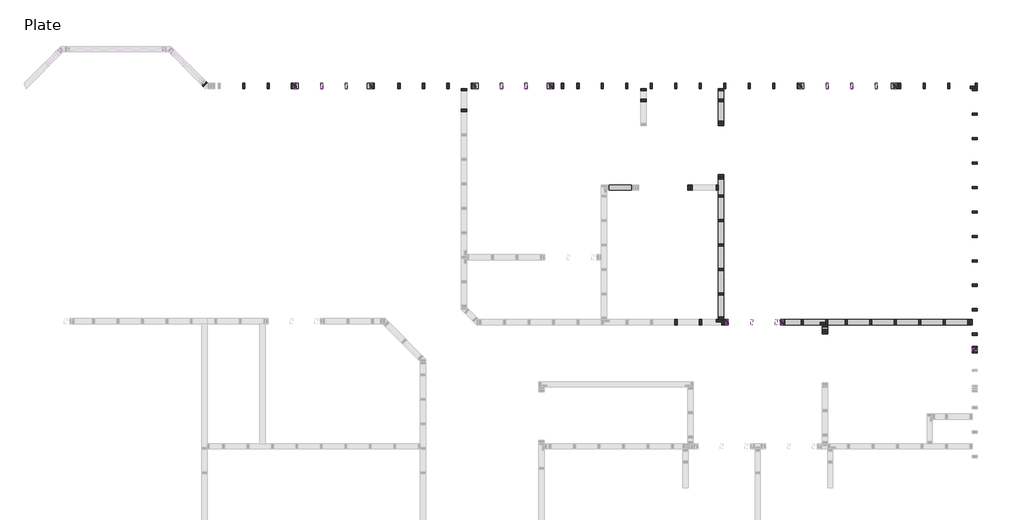
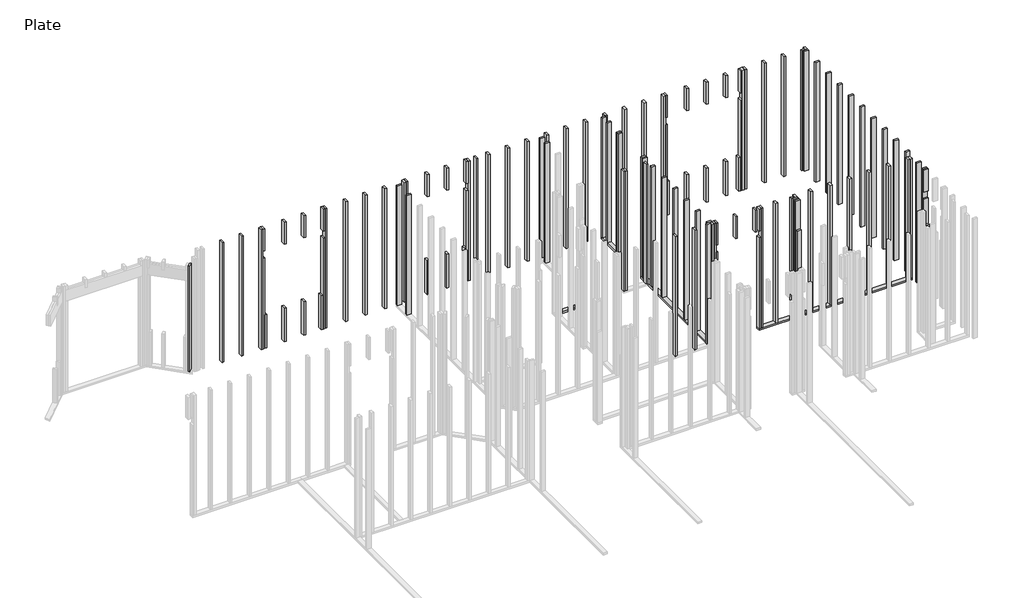
# One storey, part 5 of 5: 118 columns, 5 beams.
"""IFC4 building model written with IfcOpenShell, lengths in millimetres."""

import ifcopenshell
import ifcopenshell.guid

model = None  # the IFC model being written
_history = None  # IfcOwnerHistory: only IFC2X3 demands one
_inside = {}  # id of a spatial element -> (the spatial element, [elements in it])
_under = {}  # id of a project, library or spatial element -> (it, [spatial elements below it])
_declared = {}  # id of a project -> (the project, [libraries it declares])
_typed = {}  # id of a type object -> (the type object, [elements of that type])
_made_of = {}  # id of a material, layer set ... -> (it, [elements and type objects made of it])


def new_model(schema):
    """Start an empty IFC model of exactly this schema.

    Asked for "IFC4X3", IfcOpenShell would pick the latest addendum, in which some entities
    have other attributes; the version numbers below select the first issue.
    IFC2X3 requires an IfcOwnerHistory on every rooted entity: one is made here for all.
    """
    global model, _history
    if schema == "IFC4X3":
        model = ifcopenshell.file(schema_version=(4, 3, 0, 0))
    else:
        model = ifcopenshell.file(schema=schema)
    _inside.clear()
    _under.clear()
    _declared.clear()
    _typed.clear()
    _made_of.clear()
    _history = None
    if model.schema == "IFC2X3":
        org = make("IfcOrganization", Name="unknown")
        user = make(
            "IfcPersonAndOrganization",
            ThePerson=make("IfcPerson", FamilyName="unknown"),
            TheOrganization=org,
        )
        app = make(
            "IfcApplication",
            ApplicationDeveloper=org,
            Version="unknown",
            ApplicationFullName="unknown",
            ApplicationIdentifier="unknown",
        )
        _history = make(
            "IfcOwnerHistory",
            OwningUser=user,
            OwningApplication=app,
            ChangeAction="ADDED",
            CreationDate=0,
        )
    return model


def make(cls, **values):
    """One entity of the class cls with the attributes given. An attribute that is None is left unset."""
    return model.create_entity(
        cls, **{name: value for name, value in values.items() if value is not None}
    )


def rooted(cls, **values):
    """An entity with a GlobalId (a new one), such as an element, a storey or a relation."""
    return make(cls, GlobalId=ifcopenshell.guid.new(), OwnerHistory=_history, **values)


def si_unit(unit_type, name, prefix=None):
    """IfcSIUnit, for example si_unit("LENGTHUNIT", "METRE", prefix="MILLI")."""
    return make("IfcSIUnit", UnitType=unit_type, Prefix=prefix, Name=name)


def assignment(units):
    """IfcUnitAssignment: the units of a project."""
    return None if units is None else make("IfcUnitAssignment", Units=units)


def point(xyz):
    """IfcCartesianPoint."""
    return None if xyz is None else make("IfcCartesianPoint", Coordinates=xyz)


def direction(xyz):
    """IfcDirection."""
    return None if xyz is None else make("IfcDirection", DirectionRatios=xyz)


def frame(location, z_axis=None, x_axis=None):
    """IfcAxis2Placement3D, a coordinate frame: its origin and axes. An axis left out is left unset."""
    return make(
        "IfcAxis2Placement3D",
        Location=point(location),
        Axis=direction(z_axis),
        RefDirection=direction(x_axis),
    )


def origin():
    """The frame at (0, 0, 0) with its axes left unset."""
    return frame((0.0, 0.0, 0.0))


def place(relative_to, where):
    """IfcLocalPlacement: puts the frame where relative to a parent placement (None: the world)."""
    return make(
        "IfcLocalPlacement", PlacementRelTo=relative_to, RelativePlacement=where
    )


def context(
    kind, dimensions, precision=None, world=None, true_north=None, identifier=None
):
    """IfcGeometricRepresentationContext, for example the 3D "Model" context."""
    return make(
        "IfcGeometricRepresentationContext",
        ContextIdentifier=identifier,
        ContextType=kind,
        CoordinateSpaceDimension=dimensions,
        Precision=precision,
        WorldCoordinateSystem=world,
        TrueNorth=true_north,
    )


def project(units=None, contexts=None):
    """IfcProject with its units and contexts."""
    return rooted(
        "IfcProject",
        Name="project",
        RepresentationContexts=contexts,
        UnitsInContext=assignment(units),
    )


def spatial(cls, under=None, at=None, **own):
    """A site, building, storey or space (cls), placed at a placement, below another one or the project."""
    s = rooted(cls, ObjectPlacement=at, **own)
    if under is not None:
        _under.setdefault(under.id(), (under, []))[1].append(s)
    return s


def polyline(points):
    """IfcPolyline through the points."""
    return make("IfcPolyline", Points=[point(p) for p in points])


def outline(outer, holes=None, kind="AREA"):
    """IfcArbitraryClosedProfileDef: a profile drawn as a closed curve; with holes, ...WithVoids."""
    if holes is None:
        return make("IfcArbitraryClosedProfileDef", ProfileType=kind, OuterCurve=outer)
    return make(
        "IfcArbitraryProfileDefWithVoids",
        ProfileType=kind,
        OuterCurve=outer,
        InnerCurves=holes,
    )


def extrude(swept, where, along, depth):
    """IfcExtrudedAreaSolid: the profile swept, set in the frame where, extruded along a direction by depth."""
    return make(
        "IfcExtrudedAreaSolid",
        SweptArea=swept,
        Position=where,
        ExtrudedDirection=direction(along),
        Depth=depth,
    )


def shape(context_of_items, identifier, shape_type, items):
    """IfcShapeRepresentation: the items that make up one representation, for example the "Body"."""
    return make(
        "IfcShapeRepresentation",
        ContextOfItems=context_of_items,
        RepresentationIdentifier=identifier,
        RepresentationType=shape_type,
        Items=items,
    )


def source(mapping_origin, context_of_items, identifier, shape_type, items):
    """IfcRepresentationMap: a shape defined once, which mapped items show again and again."""
    return make(
        "IfcRepresentationMap",
        MappingOrigin=mapping_origin,
        MappedRepresentation=shape(context_of_items, identifier, shape_type, items),
    )


def transform(
    local_origin,
    x_axis=None,
    y_axis=None,
    z_axis=None,
    scale=None,
    scale2=None,
    scale3=None,
    uniform=True,
):
    """IfcCartesianTransformationOperator3D, or its non-uniform kind. x_axis, y_axis, z_axis: its Axis1, 2, 3."""
    if uniform:
        return make(
            "IfcCartesianTransformationOperator3D",
            Axis1=direction(x_axis),
            Axis2=direction(y_axis),
            LocalOrigin=point(local_origin),
            Scale=scale,
            Axis3=direction(z_axis),
        )
    return make(
        "IfcCartesianTransformationOperator3DnonUniform",
        Axis1=direction(x_axis),
        Axis2=direction(y_axis),
        LocalOrigin=point(local_origin),
        Scale=scale,
        Axis3=direction(z_axis),
        Scale2=scale2,
        Scale3=scale3,
    )


def mapped(mapping_source, mapping_target):
    """IfcMappedItem: shows the shape of a source again, moved by a transform."""
    return make(
        "IfcMappedItem", MappingSource=mapping_source, MappingTarget=mapping_target
    )


def made_of(thing, what):
    """Note that an element or type object is made of a material, layer set ...; save() writes the relation."""
    if what is not None:
        _made_of.setdefault(what.id(), (what, []))[1].append(thing)
    return thing


def element(
    cls,
    number,
    at=None,
    inside=None,
    cuts=None,
    type_object=None,
    material=None,
    context=None,
    identifier="Body",
    shape_type=None,
    held_by="IfcProductDefinitionShape",
    body=None,
    shapes=None,
    **own,
):
    """One element of the class cls, such as IfcWall. Its Tag is "e" and its number.

    at: its placement. inside: the storey or other place that contains it. cuts: it is an
    opening in that element (IfcRelVoidsElement). A single representation is given by context,
    identifier, shape_type and body (its items); several are given by shapes. held_by: the class
    of the entity that holds the representations. save() writes the other relations.
    """
    e = rooted(cls, Tag="e%d" % number, ObjectPlacement=at, **own)
    if body is not None:
        shapes = [shape(context, identifier, shape_type, body)]
    if shapes is not None:
        e.Representation = make(held_by, Representations=shapes)
    if inside is not None:
        _inside.setdefault(inside.id(), (inside, []))[1].append(e)
    if cuts is not None:
        rooted(
            "IfcRelVoidsElement", RelatingBuildingElement=cuts, RelatedOpeningElement=e
        )
    if type_object is not None:
        _typed.setdefault(type_object.id(), (type_object, []))[1].append(e)
    return made_of(e, material)


def aggregate(whole, parts):
    """IfcRelAggregates: a whole, such as a stair, and the parts it consists of."""
    return rooted("IfcRelAggregates", RelatingObject=whole, RelatedObjects=parts)


def save(model, path):
    """Write the relations noted so far, then the file.

    IfcRelAggregates (storeys below a building ...), IfcRelContainedInSpatialStructure (elements
    in a storey), IfcRelDefinesByType, IfcRelAssociatesMaterial and IfcRelDeclares: one each for
    every whole, place, type object, material and project.
    """
    for whole, parts in _under.values():
        aggregate(whole, parts)
    for where, things in _inside.values():
        rooted(
            "IfcRelContainedInSpatialStructure",
            RelatedElements=things,
            RelatingStructure=where,
        )
    for kind, things in _typed.values():
        rooted("IfcRelDefinesByType", RelatedObjects=things, RelatingType=kind)
    for what, things in _made_of.values():
        rooted("IfcRelAssociatesMaterial", RelatedObjects=things, RelatingMaterial=what)
    for by, libraries in _declared.values():
        rooted("IfcRelDeclares", RelatingContext=by, RelatedDefinitions=libraries)
    model.write(path)


def dimension_lumber_supporting_bottom_plate_83ad6fc0(model_context):
    return source(origin(), model_context, "Body", "SweptSolid", [
        extrude(outline(polyline([(1226.5374575, -44.45), (-1182.0874575, -44.45), (-1182.0874575, 44.45), (1226.5374575, 44.45), (1226.5374575, -44.45)])), frame((0.0, 0.0, -19.05), z_axis=(0.0, 0.0, 1.0), x_axis=(1.0, 0.0, 0.0)), (0.0, 0.0, 1.0), 38.1),
    ])


def dimension_lumber_supporting_bottom_plate_a6d88285(model_context):
    return source(origin(), model_context, "Body", "SweptSolid", [
        extrude(outline(polyline([(682.325, 44.45), (1216.325, 44.45), (1216.325, -44.45), (682.325, -44.45), (682.325, 44.45)])), frame((0.0, 0.0, -19.05), z_axis=(0.0, 0.0, 1.0), x_axis=(1.0, 0.0, 0.0)), (0.0, 0.0, 1.0), 38.1),
    ])


def dimension_lumber_supporting_bottom_plate_937476ce(model_context):
    return source(origin(), model_context, "Body", "SweptSolid", [
        extrude(outline(polyline([(53.975, 44.45), (53.975, -44.45), (-99.615625, -44.45), (-99.615625, 44.45), (53.975, 44.45)])), frame((0.0, 0.0, -19.05), z_axis=(0.0, 0.0, 1.0), x_axis=(1.0, 0.0, 0.0)), (0.0, 0.0, 1.0), 38.1),
    ])


def dimension_lumber_supporting_bottom_plate_42822fc3(model_context):
    return source(origin(), model_context, "Body", "SweptSolid", [
        extrude(outline(polyline([(285.5562925, -44.45), (-330.0062925, -44.45), (-330.0062925, 44.45), (285.5562925, 44.45), (285.5562925, -44.45)])), frame((0.0, 0.0, -19.05), z_axis=(0.0, 0.0, 1.0), x_axis=(1.0, 0.0, 0.0)), (0.0, 0.0, 1.0), 38.1),
    ])


def dimension_lumber_column_2x4_07183c39(model_context):
    return source(origin(), model_context, "Body", "SweptSolid", [
        extrude(outline(polyline([(19.05, 44.45), (19.05, -44.45), (-19.05, -44.45), (-19.05, 44.45), (19.05, 44.45)])), frame((0.0, 0.0, 56.35625), z_axis=(0.0, 0.0, 1.0), x_axis=(1.0, 0.0, 0.0)), (0.0, 0.0, 1.0), 2636.04375),
    ])


def dimension_lumber_column_2x4_f24b5bbb(model_context):
    return source(origin(), model_context, "Body", "SweptSolid", [
        extrude(outline(polyline([(19.05, -44.45), (-19.05, -44.45), (-19.05, 44.45), (19.05, 44.45), (19.05, -44.45)])), frame((0.0, 0.0, 56.35625), z_axis=(0.0, 0.0, 1.0), x_axis=(1.0, 0.0, 0.0)), (0.0, 0.0, 1.0), 2636.04375),
    ])


def dimension_lumber_column_2x4_0f816ddf(model_context):
    return source(origin(), model_context, "Body", "SweptSolid", [
        extrude(outline(polyline([(19.05, 44.45), (19.05, -44.45), (-19.05, -44.45), (-19.05, 44.45), (19.05, 44.45)])), frame((0.0, 0.0, 56.35625), z_axis=(0.0, 0.0, 1.0), x_axis=(1.0, 0.0, 0.0)), (0.0, 0.0, 1.0), 1999.853125),
    ])


def dimension_lumber_column_2x4_ae31bb9f(model_context):
    return source(origin(), model_context, "Body", "SweptSolid", [
        extrude(outline(polyline([(19.05, 44.45), (19.05, -44.45), (-19.05, -44.45), (-19.05, 44.45), (19.05, 44.45)])), frame((0.0, 0.0, 56.35625), z_axis=(0.0, 0.0, 1.0), x_axis=(1.0, 0.0, 0.0)), (0.0, 0.0, 1.0), 2331.24375),
    ])


def dimension_lumber_column_2x4_c2f848da(model_context):
    return source(origin(), model_context, "Body", "SweptSolid", [
        extrude(outline(polyline([(19.05, 44.45), (19.05, -44.45), (-19.05, -44.45), (-19.05, 44.45), (19.05, 44.45)])), frame((0.0, 0.0, 2208.609375), z_axis=(0.0, 0.0, 1.0), x_axis=(1.0, 0.0, 0.0)), (0.0, 0.0, 1.0), 483.790625),
    ])


def dimension_lumber_column_2x4_35883525(model_context):
    return source(origin(), model_context, "Body", "SweptSolid", [
        extrude(outline(polyline([(19.05, 44.45), (19.05, -44.45), (-19.05, -44.45), (-19.05, 44.45), (19.05, 44.45)])), frame((0.0, 0.0, 56.35625), z_axis=(0.0, 0.0, 1.0), x_axis=(1.0, 0.0, 0.0)), (0.0, 0.0, 1.0), 742.553125),
    ])


def dimension_lumber_column_2x4_c4e013fe(model_context):
    return source(origin(), model_context, "Body", "SweptSolid", [
        extrude(outline(polyline([(19.05, 44.45), (19.05, -44.45), (-19.05, -44.45), (-19.05, 44.45), (19.05, 44.45)])), frame((0.0, 0.0, 56.35625), z_axis=(0.0, 0.0, 1.0), x_axis=(1.0, 0.0, 0.0)), (0.0, 0.0, 1.0), 1444.228125),
    ])


model = new_model("IFC4")

# Units and contexts
model_context = context("Model", 3, world=origin())
ifc_project = project(units=[si_unit("LENGTHUNIT", "METRE", prefix="MILLI")], contexts=[model_context])

# Site, building, storey
site = spatial("IfcSite", under=ifc_project)
building = spatial("IfcBuilding", under=site)
storey = spatial("IfcBuildingStorey", under=building, Name="Plate", Elevation=56.35625)

# Beams
placement = place(None, origin())
element("IfcBeam", 1, ObjectType="Dimension Lumber : Supporting Bottom Plate", at=placement, inside=storey, context=model_context, shape_type="SweptSolid", body=[
    extrude(outline(polyline([(9971.0441499, 473.4459053), (9971.0441499, 562.3459053), (13155.1722749, 562.3459053), (13155.1722749, 473.4459053), (9971.0441499, 473.4459053)])), frame((0.0, 0.0, 18.25625), z_axis=(0.0, 0.0, 1.0), x_axis=(1.0, 0.0, 0.0)), (0.0, 0.0, 1.0), 38.1),
])
dimension_lumber_supporting_bottom_plate_shape = dimension_lumber_supporting_bottom_plate_83ad6fc0(model_context)
element("IfcBeam", 2, ObjectType="Dimension Lumber : Supporting Bottom Plate", at=placement, inside=storey, context=model_context, shape_type="MappedRepresentation", body=[
    mapped(dimension_lumber_supporting_bottom_plate_shape, transform((8987.9847749, 1744.4333628, 37.30625), x_axis=(0.0, 1.0, 0.0), y_axis=(-1.0, 0.0, 0.0), z_axis=(0.0, 0.0, 1.0))),
])
dimension_lumber_supporting_bottom_plate_2_shape = dimension_lumber_supporting_bottom_plate_a6d88285(model_context)
element("IfcBeam", 3, ObjectType="Dimension Lumber : Supporting Bottom Plate", at=placement, inside=storey, context=model_context, shape_type="MappedRepresentation", body=[
    mapped(dimension_lumber_supporting_bottom_plate_2_shape, transform((8305.6597749, 2753.0959053, 37.30625), x_axis=(-1.0, 0.0, 0.0), y_axis=(0.0, -1.0, 0.0), z_axis=(0.0, 0.0, 1.0))),
])
dimension_lumber_supporting_bottom_plate_3_shape = dimension_lumber_supporting_bottom_plate_937476ce(model_context)
element("IfcBeam", 4, ObjectType="Dimension Lumber : Supporting Bottom Plate", at=placement, inside=storey, context=model_context, shape_type="MappedRepresentation", body=[
    mapped(dimension_lumber_supporting_bottom_plate_3_shape, transform((10715.1847749, 419.4709053, 37.30625), x_axis=(0.0, 1.0, 0.0), y_axis=(-1.0, 0.0, 0.0), z_axis=(0.0, 0.0, 1.0))),
])
dimension_lumber_supporting_bottom_plate_4_shape = dimension_lumber_supporting_bottom_plate_42822fc3(model_context)
element("IfcBeam", 5, ObjectType="Dimension Lumber : Supporting Bottom Plate", at=placement, inside=storey, context=model_context, shape_type="MappedRepresentation", body=[
    mapped(dimension_lumber_supporting_bottom_plate_4_shape, transform((8987.9847749, 4113.7771128, 37.30625), x_axis=(0.0, 1.0, 0.0), y_axis=(-1.0, 0.0, 0.0), z_axis=(0.0, 0.0, 1.0))),
])

# Columns
dimension_lumber_column_2x4_shape = dimension_lumber_column_2x4_07183c39(model_context)
element("IfcColumn", 6, ObjectType="Dimension Lumber-Column : 2x4", at=placement, inside=storey, context=model_context, shape_type="MappedRepresentation", body=[
    mapped(dimension_lumber_column_2x4_shape, transform((13225.0222749, 4443.7834053, 0.0), x_axis=(1.0, 0.0, 0.0), y_axis=(0.0, 1.0, 0.0), z_axis=(0.0, 0.0, 1.0))),
])
element("IfcColumn", 7, ObjectType="Dimension Lumber-Column : 2x4", at=placement, inside=storey, context=model_context, shape_type="MappedRepresentation", body=[
    mapped(dimension_lumber_column_2x4_shape, transform((12767.8222749, 4443.7834053, 0.0), x_axis=(1.0, 0.0, 0.0), y_axis=(0.0, 1.0, 0.0), z_axis=(0.0, 0.0, 1.0))),
])
element("IfcColumn", 8, ObjectType="Dimension Lumber-Column : 2x4", at=placement, inside=storey, context=model_context, shape_type="MappedRepresentation", body=[
    mapped(dimension_lumber_column_2x4_shape, transform((12361.4222749, 4443.7834053, 0.0), x_axis=(1.0, 0.0, 0.0), y_axis=(0.0, 1.0, 0.0), z_axis=(0.0, 0.0, 1.0))),
])
element("IfcColumn", 9, ObjectType="Dimension Lumber-Column : 2x4", at=placement, inside=storey, context=model_context, shape_type="MappedRepresentation", body=[
    mapped(dimension_lumber_column_2x4_shape, transform((10268.3035246, 4443.7834053, 0.0), x_axis=(1.0, 0.0, 0.0), y_axis=(0.0, 1.0, 0.0), z_axis=(0.0, 0.0, 1.0))),
])
element("IfcColumn", 10, ObjectType="Dimension Lumber-Column : 2x4", at=placement, inside=storey, context=model_context, shape_type="MappedRepresentation", body=[
    mapped(dimension_lumber_column_2x4_shape, transform((9861.9035246, 4443.7834053, 0.0), x_axis=(1.0, 0.0, 0.0), y_axis=(0.0, 1.0, 0.0), z_axis=(0.0, 0.0, 1.0))),
])
element("IfcColumn", 11, ObjectType="Dimension Lumber-Column : 2x4", at=placement, inside=storey, context=model_context, shape_type="MappedRepresentation", body=[
    mapped(dimension_lumber_column_2x4_shape, transform((9455.5035246, 4443.7834053, 0.0), x_axis=(1.0, 0.0, 0.0), y_axis=(0.0, 1.0, 0.0), z_axis=(0.0, 0.0, 1.0))),
])
element("IfcColumn", 12, ObjectType="Dimension Lumber-Column : 2x4", at=placement, inside=storey, context=model_context, shape_type="MappedRepresentation", body=[
    mapped(dimension_lumber_column_2x4_shape, transform((9049.1035246, 4443.7834053, 0.0), x_axis=(1.0, 0.0, 0.0), y_axis=(0.0, 1.0, 0.0), z_axis=(0.0, 0.0, 1.0))),
])
element("IfcColumn", 13, ObjectType="Dimension Lumber-Column : 2x4", at=placement, inside=storey, context=model_context, shape_type="MappedRepresentation", body=[
    mapped(dimension_lumber_column_2x4_shape, transform((8642.7035246, 4443.7834053, 0.0), x_axis=(1.0, 0.0, 0.0), y_axis=(0.0, 1.0, 0.0), z_axis=(0.0, 0.0, 1.0))),
])
element("IfcColumn", 14, ObjectType="Dimension Lumber-Column : 2x4", at=placement, inside=storey, context=model_context, shape_type="MappedRepresentation", body=[
    mapped(dimension_lumber_column_2x4_shape, transform((8236.3035246, 4443.7834053, 0.0), x_axis=(1.0, 0.0, 0.0), y_axis=(0.0, 1.0, 0.0), z_axis=(0.0, 0.0, 1.0))),
])
element("IfcColumn", 15, ObjectType="Dimension Lumber-Column : 2x4", at=placement, inside=storey, context=model_context, shape_type="MappedRepresentation", body=[
    mapped(dimension_lumber_column_2x4_shape, transform((7829.9035246, 4443.7834053, 0.0), x_axis=(1.0, 0.0, 0.0), y_axis=(0.0, 1.0, 0.0), z_axis=(0.0, 0.0, 1.0))),
])
element("IfcColumn", 16, ObjectType="Dimension Lumber-Column : 2x4", at=placement, inside=storey, context=model_context, shape_type="MappedRepresentation", body=[
    mapped(dimension_lumber_column_2x4_shape, transform((7423.5035246, 4443.7834053, 0.0), x_axis=(1.0, 0.0, 0.0), y_axis=(0.0, 1.0, 0.0), z_axis=(0.0, 0.0, 1.0))),
])
element("IfcColumn", 17, ObjectType="Dimension Lumber-Column : 2x4", at=placement, inside=storey, context=model_context, shape_type="MappedRepresentation", body=[
    mapped(dimension_lumber_column_2x4_shape, transform((7017.1035246, 4443.7834053, 0.0), x_axis=(1.0, 0.0, 0.0), y_axis=(0.0, 1.0, 0.0), z_axis=(0.0, 0.0, 1.0))),
])
element("IfcColumn", 18, ObjectType="Dimension Lumber-Column : 2x4", at=placement, inside=storey, context=model_context, shape_type="MappedRepresentation", body=[
    mapped(dimension_lumber_column_2x4_shape, transform((6610.7035246, 4443.7834053, 0.0), x_axis=(1.0, 0.0, 0.0), y_axis=(0.0, 1.0, 0.0), z_axis=(0.0, 0.0, 1.0))),
])
element("IfcColumn", 19, ObjectType="Dimension Lumber-Column : 2x4", at=placement, inside=storey, context=model_context, shape_type="MappedRepresentation", body=[
    mapped(dimension_lumber_column_2x4_shape, transform((6356.7035249, 4443.7834053, 0.0), x_axis=(1.0, 0.0, 0.0), y_axis=(0.0, 1.0, 0.0), z_axis=(0.0, 0.0, 1.0))),
])
element("IfcColumn", 20, ObjectType="Dimension Lumber-Column : 2x4", at=placement, inside=storey, context=model_context, shape_type="MappedRepresentation", body=[
    mapped(dimension_lumber_column_2x4_shape, transform((4860.4847743, 4443.7834053, 0.0), x_axis=(1.0, 0.0, 0.0), y_axis=(0.0, 1.0, 0.0), z_axis=(0.0, 0.0, 1.0))),
])
element("IfcColumn", 21, ObjectType="Dimension Lumber-Column : 2x4", at=placement, inside=storey, context=model_context, shape_type="MappedRepresentation", body=[
    mapped(dimension_lumber_column_2x4_shape, transform((4454.0847743, 4443.7834053, 0.0), x_axis=(1.0, 0.0, 0.0), y_axis=(0.0, 1.0, 0.0), z_axis=(0.0, 0.0, 1.0))),
])
element("IfcColumn", 22, ObjectType="Dimension Lumber-Column : 2x4", at=placement, inside=storey, context=model_context, shape_type="MappedRepresentation", body=[
    mapped(dimension_lumber_column_2x4_shape, transform((4047.6847743, 4443.7834053, 0.0), x_axis=(1.0, 0.0, 0.0), y_axis=(0.0, 1.0, 0.0), z_axis=(0.0, 0.0, 1.0))),
])
element("IfcColumn", 23, ObjectType="Dimension Lumber-Column : 2x4", at=placement, inside=storey, context=model_context, shape_type="MappedRepresentation", body=[
    mapped(dimension_lumber_column_2x4_shape, transform((3641.2847743, 4443.7834053, 0.0), x_axis=(1.0, 0.0, 0.0), y_axis=(0.0, 1.0, 0.0), z_axis=(0.0, 0.0, 1.0))),
])
element("IfcColumn", 24, ObjectType="Dimension Lumber-Column : 2x4", at=placement, inside=storey, context=model_context, shape_type="MappedRepresentation", body=[
    mapped(dimension_lumber_column_2x4_shape, transform((1875.9847743, 4443.7834053, 0.0), x_axis=(1.0, 0.0, 0.0), y_axis=(0.0, 1.0, 0.0), z_axis=(0.0, 0.0, 1.0))),
])
element("IfcColumn", 25, ObjectType="Dimension Lumber-Column : 2x4", at=placement, inside=storey, context=model_context, shape_type="MappedRepresentation", body=[
    mapped(dimension_lumber_column_2x4_shape, transform((1469.5847743, 4443.7834053, 0.0), x_axis=(1.0, 0.0, 0.0), y_axis=(0.0, 1.0, 0.0), z_axis=(0.0, 0.0, 1.0))),
])
element("IfcColumn", 26, ObjectType="Dimension Lumber-Column : 2x4", at=placement, inside=storey, context=model_context, shape_type="MappedRepresentation", body=[
    mapped(dimension_lumber_column_2x4_shape, transform((1063.1847743, 4443.7834053, 0.0), x_axis=(1.0, 0.0, 0.0), y_axis=(0.0, 1.0, 0.0), z_axis=(0.0, 0.0, 1.0))),
])
element("IfcColumn", 27, ObjectType="Dimension Lumber-Column : 2x4", at=placement, inside=storey, context=model_context, shape_type="MappedRepresentation", body=[
    mapped(dimension_lumber_column_2x4_shape, transform((13199.6222749, 3973.8834053, 0.0), x_axis=(0.0, 1.0, 0.0), y_axis=(-1.0, 0.0, 0.0), z_axis=(0.0, 0.0, 1.0))),
])
element("IfcColumn", 28, ObjectType="Dimension Lumber-Column : 2x4", at=placement, inside=storey, context=model_context, shape_type="MappedRepresentation", body=[
    mapped(dimension_lumber_column_2x4_shape, transform((13199.6222749, 3567.4834053, 0.0), x_axis=(0.0, 1.0, 0.0), y_axis=(-1.0, 0.0, 0.0), z_axis=(0.0, 0.0, 1.0))),
])
element("IfcColumn", 29, ObjectType="Dimension Lumber-Column : 2x4", at=placement, inside=storey, context=model_context, shape_type="MappedRepresentation", body=[
    mapped(dimension_lumber_column_2x4_shape, transform((13199.6222749, 3161.0834053, 0.0), x_axis=(0.0, 1.0, 0.0), y_axis=(-1.0, 0.0, 0.0), z_axis=(0.0, 0.0, 1.0))),
])
element("IfcColumn", 30, ObjectType="Dimension Lumber-Column : 2x4", at=placement, inside=storey, context=model_context, shape_type="MappedRepresentation", body=[
    mapped(dimension_lumber_column_2x4_shape, transform((13199.6222749, 2754.6834053, 0.0), x_axis=(0.0, 1.0, 0.0), y_axis=(-1.0, 0.0, 0.0), z_axis=(0.0, 0.0, 1.0))),
])
element("IfcColumn", 31, ObjectType="Dimension Lumber-Column : 2x4", at=placement, inside=storey, context=model_context, shape_type="MappedRepresentation", body=[
    mapped(dimension_lumber_column_2x4_shape, transform((13199.6222749, 2348.2834053, 0.0), x_axis=(0.0, 1.0, 0.0), y_axis=(-1.0, 0.0, 0.0), z_axis=(0.0, 0.0, 1.0))),
])
element("IfcColumn", 32, ObjectType="Dimension Lumber-Column : 2x4", at=placement, inside=storey, context=model_context, shape_type="MappedRepresentation", body=[
    mapped(dimension_lumber_column_2x4_shape, transform((13199.6222749, 1941.8834053, 0.0), x_axis=(0.0, 1.0, 0.0), y_axis=(-1.0, 0.0, 0.0), z_axis=(0.0, 0.0, 1.0))),
])
element("IfcColumn", 33, ObjectType="Dimension Lumber-Column : 2x4", at=placement, inside=storey, context=model_context, shape_type="MappedRepresentation", body=[
    mapped(dimension_lumber_column_2x4_shape, transform((13199.6222749, 1535.4834053, 0.0), x_axis=(0.0, 1.0, 0.0), y_axis=(-1.0, 0.0, 0.0), z_axis=(0.0, 0.0, 1.0))),
])
element("IfcColumn", 34, ObjectType="Dimension Lumber-Column : 2x4", at=placement, inside=storey, context=model_context, shape_type="MappedRepresentation", body=[
    mapped(dimension_lumber_column_2x4_shape, transform((13199.6222749, 1129.0834053, 0.0), x_axis=(0.0, 1.0, 0.0), y_axis=(-1.0, 0.0, 0.0), z_axis=(0.0, 0.0, 1.0))),
])
element("IfcColumn", 35, ObjectType="Dimension Lumber-Column : 2x4", at=placement, inside=storey, context=model_context, shape_type="MappedRepresentation", body=[
    mapped(dimension_lumber_column_2x4_shape, transform((13199.6222749, 722.6834053, 0.0), x_axis=(0.0, 1.0, 0.0), y_axis=(-1.0, 0.0, 0.0), z_axis=(0.0, 0.0, 1.0))),
])
element("IfcColumn", 36, ObjectType="Dimension Lumber-Column : 2x4", at=placement, inside=storey, context=model_context, shape_type="MappedRepresentation", body=[
    mapped(dimension_lumber_column_2x4_shape, transform((13199.6222749, 316.2834053, 0.0), x_axis=(0.0, 1.0, 0.0), y_axis=(-1.0, 0.0, 0.0), z_axis=(0.0, 0.0, 1.0))),
])
element("IfcColumn", 37, ObjectType="Dimension Lumber-Column : 2x4", at=placement, inside=storey, context=model_context, shape_type="MappedRepresentation", body=[
    mapped(dimension_lumber_column_2x4_shape, transform((13199.6222749, 98.7959053, 0.0), x_axis=(0.0, 1.0, 0.0), y_axis=(-1.0, 0.0, 0.0), z_axis=(0.0, 0.0, 1.0))),
])
element("IfcColumn", 38, ObjectType="Dimension Lumber-Column : 2x4", at=placement, inside=storey, context=model_context, shape_type="MappedRepresentation", body=[
    mapped(dimension_lumber_column_2x4_shape, transform((13199.6222749, 4380.2834053, 0.0), x_axis=(0.0, 1.0, 0.0), y_axis=(-1.0, 0.0, 0.0), z_axis=(0.0, 0.0, 1.0))),
])
element("IfcColumn", 39, ObjectType="Dimension Lumber-Column : 2x4", at=placement, inside=storey, context=model_context, shape_type="MappedRepresentation", body=[
    mapped(dimension_lumber_column_2x4_shape, transform((13136.1222749, 517.8959053, 0.0), x_axis=(1.0, 0.0, 0.0), y_axis=(0.0, 1.0, 0.0), z_axis=(0.0, 0.0, 1.0))),
])
element("IfcColumn", 40, ObjectType="Dimension Lumber-Column : 2x4", at=placement, inside=storey, context=model_context, shape_type="MappedRepresentation", body=[
    mapped(dimension_lumber_column_2x4_shape, transform((13098.0222749, 517.8959053, 0.0), x_axis=(1.0, 0.0, 0.0), y_axis=(0.0, 1.0, 0.0), z_axis=(0.0, 0.0, 1.0))),
])
element("IfcColumn", 41, ObjectType="Dimension Lumber-Column : 2x4", at=placement, inside=storey, context=model_context, shape_type="MappedRepresentation", body=[
    mapped(dimension_lumber_column_2x4_shape, transform((12691.6222749, 517.8959053, 0.0), x_axis=(1.0, 0.0, 0.0), y_axis=(0.0, 1.0, 0.0), z_axis=(0.0, 0.0, 1.0))),
])
element("IfcColumn", 42, ObjectType="Dimension Lumber-Column : 2x4", at=placement, inside=storey, context=model_context, shape_type="MappedRepresentation", body=[
    mapped(dimension_lumber_column_2x4_shape, transform((12285.2222749, 517.8959053, 0.0), x_axis=(1.0, 0.0, 0.0), y_axis=(0.0, 1.0, 0.0), z_axis=(0.0, 0.0, 1.0))),
])
element("IfcColumn", 43, ObjectType="Dimension Lumber-Column : 2x4", at=placement, inside=storey, context=model_context, shape_type="MappedRepresentation", body=[
    mapped(dimension_lumber_column_2x4_shape, transform((11878.8222749, 517.8959053, 0.0), x_axis=(1.0, 0.0, 0.0), y_axis=(0.0, 1.0, 0.0), z_axis=(0.0, 0.0, 1.0))),
])
element("IfcColumn", 44, ObjectType="Dimension Lumber-Column : 2x4", at=placement, inside=storey, context=model_context, shape_type="MappedRepresentation", body=[
    mapped(dimension_lumber_column_2x4_shape, transform((11472.4222749, 517.8959053, 0.0), x_axis=(1.0, 0.0, 0.0), y_axis=(0.0, 1.0, 0.0), z_axis=(0.0, 0.0, 1.0))),
])
element("IfcColumn", 45, ObjectType="Dimension Lumber-Column : 2x4", at=placement, inside=storey, context=model_context, shape_type="MappedRepresentation", body=[
    mapped(dimension_lumber_column_2x4_shape, transform((11066.0222749, 517.8959053, 0.0), x_axis=(1.0, 0.0, 0.0), y_axis=(0.0, 1.0, 0.0), z_axis=(0.0, 0.0, 1.0))),
])
element("IfcColumn", 46, ObjectType="Dimension Lumber-Column : 2x4", at=placement, inside=storey, context=model_context, shape_type="MappedRepresentation", body=[
    mapped(dimension_lumber_column_2x4_shape, transform((10742.1722749, 517.8959053, 0.0), x_axis=(1.0, 0.0, 0.0), y_axis=(0.0, 1.0, 0.0), z_axis=(0.0, 0.0, 1.0))),
])
element("IfcColumn", 47, ObjectType="Dimension Lumber-Column : 2x4", at=placement, inside=storey, context=model_context, shape_type="MappedRepresentation", body=[
    mapped(dimension_lumber_column_2x4_shape, transform((10335.7722749, 517.8959053, 0.0), x_axis=(1.0, 0.0, 0.0), y_axis=(0.0, 1.0, 0.0), z_axis=(0.0, 0.0, 1.0))),
])
element("IfcColumn", 48, ObjectType="Dimension Lumber-Column : 2x4", at=placement, inside=storey, context=model_context, shape_type="MappedRepresentation", body=[
    mapped(dimension_lumber_column_2x4_shape, transform((8646.2753999, 517.8959053, 0.0), x_axis=(1.0, 0.0, 0.0), y_axis=(0.0, 1.0, 0.0), z_axis=(0.0, 0.0, 1.0))),
])
element("IfcColumn", 49, ObjectType="Dimension Lumber-Column : 2x4", at=placement, inside=storey, context=model_context, shape_type="MappedRepresentation", body=[
    mapped(dimension_lumber_column_2x4_shape, transform((8239.8753999, 517.8959053, 0.0), x_axis=(1.0, 0.0, 0.0), y_axis=(0.0, 1.0, 0.0), z_axis=(0.0, 0.0, 1.0))),
])
element("IfcColumn", 50, ObjectType="Dimension Lumber-Column : 2x4", at=placement, inside=storey, context=model_context, shape_type="MappedRepresentation", body=[
    mapped(dimension_lumber_column_2x4_shape, transform((10028.1941499, 517.8959053, 0.0), x_axis=(1.0, 0.0, 0.0), y_axis=(0.0, 1.0, 0.0), z_axis=(0.0, 0.0, 1.0))),
])
element("IfcColumn", 51, ObjectType="Dimension Lumber-Column : 2x4", at=placement, inside=storey, context=model_context, shape_type="MappedRepresentation", body=[
    mapped(dimension_lumber_column_2x4_shape, transform((9052.6753999, 517.8959053, 0.0), x_axis=(1.0, 0.0, 0.0), y_axis=(0.0, 1.0, 0.0), z_axis=(0.0, 0.0, 1.0))),
])
element("IfcColumn", 52, ObjectType="Dimension Lumber-Column : 2x4", at=placement, inside=storey, context=model_context, shape_type="MappedRepresentation", body=[
    mapped(dimension_lumber_column_2x4_shape, transform((13167.8722749, 4418.3834053, 0.0), x_axis=(0.0, 1.0, 0.0), y_axis=(-1.0, 0.0, 0.0), z_axis=(0.0, 0.0, 1.0))),
])
element("IfcColumn", 53, ObjectType="Dimension Lumber-Column : 2x4", at=placement, inside=storey, context=model_context, shape_type="MappedRepresentation", body=[
    mapped(dimension_lumber_column_2x4_shape, transform((11955.0222749, 4443.7834053, 0.0), x_axis=(1.0, 0.0, 0.0), y_axis=(0.0, 1.0, 0.0), z_axis=(0.0, 0.0, 1.0))),
])
element("IfcColumn", 54, ObjectType="Dimension Lumber-Column : 2x4", at=placement, inside=storey, context=model_context, shape_type="MappedRepresentation", body=[
    mapped(dimension_lumber_column_2x4_shape, transform((11906.6035252, 4443.7834053, 0.0), x_axis=(1.0, 0.0, 0.0), y_axis=(0.0, 1.0, 0.0), z_axis=(0.0, 0.0, 1.0))),
])
element("IfcColumn", 55, ObjectType="Dimension Lumber-Column : 2x4", at=placement, inside=storey, context=model_context, shape_type="MappedRepresentation", body=[
    mapped(dimension_lumber_column_2x4_shape, transform((6193.9847743, 4443.7834053, 0.0), x_axis=(1.0, 0.0, 0.0), y_axis=(0.0, 1.0, 0.0), z_axis=(0.0, 0.0, 1.0))),
])
element("IfcColumn", 56, ObjectType="Dimension Lumber-Column : 2x4", at=placement, inside=storey, context=model_context, shape_type="MappedRepresentation", body=[
    mapped(dimension_lumber_column_2x4_shape, transform((3209.4847743, 4443.7834053, 0.0), x_axis=(1.0, 0.0, 0.0), y_axis=(0.0, 1.0, 0.0), z_axis=(0.0, 0.0, 1.0))),
])
element("IfcColumn", 57, ObjectType="Dimension Lumber-Column : 2x4", at=placement, inside=storey, context=model_context, shape_type="MappedRepresentation", body=[
    mapped(dimension_lumber_column_2x4_shape, transform((8987.9847749, 3802.8208204, 0.0), x_axis=(0.0, -1.0, 0.0), y_axis=(1.0, 0.0, 0.0), z_axis=(0.0, 0.0, 1.0))),
])
element("IfcColumn", 58, ObjectType="Dimension Lumber-Column : 2x4", at=placement, inside=storey, context=model_context, shape_type="MappedRepresentation", body=[
    mapped(dimension_lumber_column_2x4_shape, transform((8987.9847749, 3840.9208204, 0.0), x_axis=(0.0, -1.0, 0.0), y_axis=(1.0, 0.0, 0.0), z_axis=(0.0, 0.0, 1.0))),
])
element("IfcColumn", 59, ObjectType="Dimension Lumber-Column : 2x4", at=placement, inside=storey, context=model_context, shape_type="MappedRepresentation", body=[
    mapped(dimension_lumber_column_2x4_shape, transform((8987.9847749, 4202.1834053, 0.0), x_axis=(0.0, -1.0, 0.0), y_axis=(1.0, 0.0, 0.0), z_axis=(0.0, 0.0, 1.0))),
])
element("IfcColumn", 60, ObjectType="Dimension Lumber-Column : 2x4", at=placement, inside=storey, context=model_context, shape_type="MappedRepresentation", body=[
    mapped(dimension_lumber_column_2x4_shape, transform((8987.9847749, 4380.2834053, 0.0), x_axis=(0.0, -1.0, 0.0), y_axis=(1.0, 0.0, 0.0), z_axis=(0.0, 0.0, 1.0))),
])
element("IfcColumn", 61, ObjectType="Dimension Lumber-Column : 2x4", at=placement, inside=storey, context=model_context, shape_type="MappedRepresentation", body=[
    mapped(dimension_lumber_column_2x4_shape, transform((7698.9347749, 4202.1834053, 0.0), x_axis=(0.0, -1.0, 0.0), y_axis=(1.0, 0.0, 0.0), z_axis=(0.0, 0.0, 1.0))),
])
element("IfcColumn", 62, ObjectType="Dimension Lumber-Column : 2x4", at=placement, inside=storey, context=model_context, shape_type="MappedRepresentation", body=[
    mapped(dimension_lumber_column_2x4_shape, transform((7698.9347749, 4380.2834053, 0.0), x_axis=(0.0, -1.0, 0.0), y_axis=(1.0, 0.0, 0.0), z_axis=(0.0, 0.0, 1.0))),
])
element("IfcColumn", 63, ObjectType="Dimension Lumber-Column : 2x4", at=placement, inside=storey, context=model_context, shape_type="MappedRepresentation", body=[
    mapped(dimension_lumber_column_2x4_shape, transform((10715.1847749, 377.0052803, 0.0), x_axis=(0.0, 1.0, 0.0), y_axis=(-1.0, 0.0, 0.0), z_axis=(0.0, 0.0, 1.0))),
])
element("IfcColumn", 64, ObjectType="Dimension Lumber-Column : 2x4", at=placement, inside=storey, context=model_context, shape_type="MappedRepresentation", body=[
    mapped(dimension_lumber_column_2x4_shape, transform((10715.1847749, 454.3959053, 0.0), x_axis=(0.0, 1.0, 0.0), y_axis=(-1.0, 0.0, 0.0), z_axis=(0.0, 0.0, 1.0))),
])
element("IfcColumn", 65, ObjectType="Dimension Lumber-Column : 2x4", at=placement, inside=storey, context=model_context, shape_type="MappedRepresentation", body=[
    mapped(dimension_lumber_column_2x4_shape, transform((10678.6722749, 492.4959053, 0.0), x_axis=(0.0, 1.0, 0.0), y_axis=(-1.0, 0.0, 0.0), z_axis=(0.0, 0.0, 1.0))),
])
element("IfcColumn", 66, ObjectType="Dimension Lumber-Column : 2x4", at=placement, inside=storey, context=model_context, shape_type="MappedRepresentation", body=[
    mapped(dimension_lumber_column_2x4_shape, transform((9014.5753999, 517.8959053, 0.0), x_axis=(1.0, 0.0, 0.0), y_axis=(0.0, 1.0, 0.0), z_axis=(0.0, 0.0, 1.0))),
])
dimension_lumber_column_2x4_2_shape = dimension_lumber_column_2x4_f24b5bbb(model_context)
element("IfcColumn", 67, ObjectType="Dimension Lumber-Column : 2x4", at=placement, inside=storey, context=model_context, shape_type="MappedRepresentation", body=[
    mapped(dimension_lumber_column_2x4_2_shape, transform((8987.9847749, 581.3959053, 0.0), x_axis=(0.0, 1.0, 0.0), y_axis=(-1.0, 0.0, 0.0), z_axis=(0.0, 0.0, 1.0))),
])
element("IfcColumn", 68, ObjectType="Dimension Lumber-Column : 2x4", at=placement, inside=storey, context=model_context, shape_type="MappedRepresentation", body=[
    mapped(dimension_lumber_column_2x4_2_shape, transform((8987.9847749, 987.7959053, 0.0), x_axis=(0.0, 1.0, 0.0), y_axis=(-1.0, 0.0, 0.0), z_axis=(0.0, 0.0, 1.0))),
])
element("IfcColumn", 69, ObjectType="Dimension Lumber-Column : 2x4", at=placement, inside=storey, context=model_context, shape_type="MappedRepresentation", body=[
    mapped(dimension_lumber_column_2x4_2_shape, transform((8987.9847749, 1394.1959053, 0.0), x_axis=(0.0, 1.0, 0.0), y_axis=(-1.0, 0.0, 0.0), z_axis=(0.0, 0.0, 1.0))),
])
element("IfcColumn", 70, ObjectType="Dimension Lumber-Column : 2x4", at=placement, inside=storey, context=model_context, shape_type="MappedRepresentation", body=[
    mapped(dimension_lumber_column_2x4_2_shape, transform((8987.9847749, 1800.5959053, 0.0), x_axis=(0.0, 1.0, 0.0), y_axis=(-1.0, 0.0, 0.0), z_axis=(0.0, 0.0, 1.0))),
])
element("IfcColumn", 71, ObjectType="Dimension Lumber-Column : 2x4", at=placement, inside=storey, context=model_context, shape_type="MappedRepresentation", body=[
    mapped(dimension_lumber_column_2x4_2_shape, transform((8987.9847749, 2206.9959053, 0.0), x_axis=(0.0, 1.0, 0.0), y_axis=(-1.0, 0.0, 0.0), z_axis=(0.0, 0.0, 1.0))),
])
element("IfcColumn", 72, ObjectType="Dimension Lumber-Column : 2x4", at=placement, inside=storey, context=model_context, shape_type="MappedRepresentation", body=[
    mapped(dimension_lumber_column_2x4_2_shape, transform((8987.9847749, 2613.3959053, 0.0), x_axis=(0.0, 1.0, 0.0), y_axis=(-1.0, 0.0, 0.0), z_axis=(0.0, 0.0, 1.0))),
])
element("IfcColumn", 73, ObjectType="Dimension Lumber-Column : 2x4", at=placement, inside=storey, context=model_context, shape_type="MappedRepresentation", body=[
    mapped(dimension_lumber_column_2x4_2_shape, transform((8951.0753999, 543.2910129, 0.0), x_axis=(0.0, 1.0, 0.0), y_axis=(-1.0, 0.0, 0.0), z_axis=(0.0, 0.0, 1.0))),
])
element("IfcColumn", 74, ObjectType="Dimension Lumber-Column : 2x4", at=placement, inside=storey, context=model_context, shape_type="MappedRepresentation", body=[
    mapped(dimension_lumber_column_2x4_2_shape, transform((8455.1847749, 2753.0959053, 0.0), x_axis=(-1.0, 0.0, 0.0), y_axis=(0.0, -1.0, 0.0), z_axis=(0.0, 0.0, 1.0))),
])
element("IfcColumn", 75, ObjectType="Dimension Lumber-Column : 2x4", at=placement, inside=storey, context=model_context, shape_type="MappedRepresentation", body=[
    mapped(dimension_lumber_column_2x4_2_shape, transform((8493.2847749, 2753.0959053, 0.0), x_axis=(-1.0, 0.0, 0.0), y_axis=(0.0, -1.0, 0.0), z_axis=(0.0, 0.0, 1.0))),
])
element("IfcColumn", 76, ObjectType="Dimension Lumber-Column : 2x4", at=placement, inside=storey, context=model_context, shape_type="MappedRepresentation", body=[
    mapped(dimension_lumber_column_2x4_2_shape, transform((8924.4847749, 2753.0959053, 0.0), x_axis=(-1.0, 0.0, 0.0), y_axis=(0.0, -1.0, 0.0), z_axis=(0.0, 0.0, 1.0))),
])
element("IfcColumn", 77, ObjectType="Dimension Lumber-Column : 2x4", at=placement, inside=storey, context=model_context, shape_type="MappedRepresentation", body=[
    mapped(dimension_lumber_column_2x4_2_shape, transform((4720.7847749, 4035.8732039, 0.0), x_axis=(0.0, 1.0, 0.0), y_axis=(-1.0, 0.0, 0.0), z_axis=(0.0, 0.0, 1.0))),
])
element("IfcColumn", 78, ObjectType="Dimension Lumber-Column : 2x4", at=placement, inside=storey, context=model_context, shape_type="MappedRepresentation", body=[
    mapped(dimension_lumber_column_2x4_2_shape, transform((4720.7847749, 4380.2834053, 0.0), x_axis=(0.0, 1.0, 0.0), y_axis=(-1.0, 0.0, 0.0), z_axis=(0.0, 0.0, 1.0))),
])
element("IfcColumn", 79, ObjectType="Dimension Lumber-Column : 2x4", at=placement, inside=storey, context=model_context, shape_type="MappedRepresentation", body=[
    mapped(dimension_lumber_column_2x4_2_shape, transform((8987.9847749, 2951.9208204, 0.0), x_axis=(0.0, 1.0, 0.0), y_axis=(-1.0, 0.0, 0.0), z_axis=(0.0, 0.0, 1.0))),
])
element("IfcColumn", 80, ObjectType="Dimension Lumber-Column : 2x4", at=placement, inside=storey, context=model_context, shape_type="MappedRepresentation", body=[
    mapped(dimension_lumber_column_2x4_2_shape, transform((8987.9847749, 2913.8208204, 0.0), x_axis=(0.0, 1.0, 0.0), y_axis=(-1.0, 0.0, 0.0), z_axis=(0.0, 0.0, 1.0))),
])
dimension_lumber_column_2x4_3_shape = dimension_lumber_column_2x4_0f816ddf(model_context)
element("IfcColumn", 81, ObjectType="Dimension Lumber-Column : 2x4", at=placement, inside=storey, context=model_context, shape_type="MappedRepresentation", body=[
    mapped(dimension_lumber_column_2x4_3_shape, transform((6155.8847743, 4443.7834053, 0.0), x_axis=(1.0, 0.0, 0.0), y_axis=(0.0, 1.0, 0.0), z_axis=(0.0, 0.0, 1.0))),
])
element("IfcColumn", 82, ObjectType="Dimension Lumber-Column : 2x4", at=placement, inside=storey, context=model_context, shape_type="MappedRepresentation", body=[
    mapped(dimension_lumber_column_2x4_3_shape, transform((4898.5847743, 4443.7834053, 0.0), x_axis=(1.0, 0.0, 0.0), y_axis=(0.0, 1.0, 0.0), z_axis=(0.0, 0.0, 1.0))),
])
element("IfcColumn", 83, ObjectType="Dimension Lumber-Column : 2x4", at=placement, inside=storey, context=model_context, shape_type="MappedRepresentation", body=[
    mapped(dimension_lumber_column_2x4_3_shape, transform((3171.3847743, 4443.7834053, 0.0), x_axis=(1.0, 0.0, 0.0), y_axis=(0.0, 1.0, 0.0), z_axis=(0.0, 0.0, 1.0))),
])
element("IfcColumn", 84, ObjectType="Dimension Lumber-Column : 2x4", at=placement, inside=storey, context=model_context, shape_type="MappedRepresentation", body=[
    mapped(dimension_lumber_column_2x4_3_shape, transform((1914.0847743, 4443.7834053, 0.0), x_axis=(1.0, 0.0, 0.0), y_axis=(0.0, 1.0, 0.0), z_axis=(0.0, 0.0, 1.0))),
])
element("IfcColumn", 85, ObjectType="Dimension Lumber-Column : 2x4", at=placement, inside=storey, context=model_context, shape_type="MappedRepresentation", body=[
    mapped(dimension_lumber_column_2x4_3_shape, transform((11868.5035252, 4443.7834053, 0.0), x_axis=(1.0, 0.0, 0.0), y_axis=(0.0, 1.0, 0.0), z_axis=(0.0, 0.0, 1.0))),
])
element("IfcColumn", 86, ObjectType="Dimension Lumber-Column : 2x4", at=placement, inside=storey, context=model_context, shape_type="MappedRepresentation", body=[
    mapped(dimension_lumber_column_2x4_3_shape, transform((10306.4035246, 4443.7834053, 0.0), x_axis=(1.0, 0.0, 0.0), y_axis=(0.0, 1.0, 0.0), z_axis=(0.0, 0.0, 1.0))),
])
element("IfcColumn", 87, ObjectType="Dimension Lumber-Column : 2x4", at=placement, inside=storey, context=model_context, shape_type="MappedRepresentation", body=[
    mapped(dimension_lumber_column_2x4_3_shape, transform((13199.6222749, 60.6959053, 0.0), x_axis=(0.0, -1.0, 0.0), y_axis=(1.0, 0.0, 0.0), z_axis=(0.0, 0.0, 1.0))),
])
dimension_lumber_column_2x4_4_shape = dimension_lumber_column_2x4_ae31bb9f(model_context)
element("IfcColumn", 88, ObjectType="Dimension Lumber-Column : 2x4", at=placement, inside=storey, context=model_context, shape_type="MappedRepresentation", body=[
    mapped(dimension_lumber_column_2x4_4_shape, transform((411.3444463, 4478.7244411, 0.0), x_axis=(0.7071067811865507, -0.7071067811865445, 0.0), y_axis=(0.7071067811865445, 0.7071067811865507, 0.0), z_axis=(0.0, 0.0, 1.0))),
])
element("IfcColumn", 89, ObjectType="Dimension Lumber-Column : 2x4", at=placement, inside=storey, context=model_context, shape_type="MappedRepresentation", body=[
    mapped(dimension_lumber_column_2x4_3_shape, transform((9990.0941499, 517.8959053, 0.0), x_axis=(1.0, 0.0, 0.0), y_axis=(0.0, 1.0, 0.0), z_axis=(0.0, 0.0, 1.0))),
])
element("IfcColumn", 90, ObjectType="Dimension Lumber-Column : 2x4", at=placement, inside=storey, context=model_context, shape_type="MappedRepresentation", body=[
    mapped(dimension_lumber_column_2x4_3_shape, transform((9090.7753999, 517.8959053, 0.0), x_axis=(1.0, 0.0, 0.0), y_axis=(0.0, 1.0, 0.0), z_axis=(0.0, 0.0, 1.0))),
])
element("IfcColumn", 91, ObjectType="Dimension Lumber-Column : 2x4", at=placement, inside=storey, context=model_context, shape_type="MappedRepresentation", body=[
    mapped(dimension_lumber_column_2x4_3_shape, transform((10715.1847749, 338.9052803, 0.0), x_axis=(0.0, 1.0, 0.0), y_axis=(-1.0, 0.0, 0.0), z_axis=(0.0, 0.0, 1.0))),
])
dimension_lumber_column_2x4_5_shape = dimension_lumber_column_2x4_c2f848da(model_context)
element("IfcColumn", 92, ObjectType="Dimension Lumber-Column : 2x4", at=placement, inside=storey, context=model_context, shape_type="MappedRepresentation", body=[
    mapped(dimension_lumber_column_2x4_5_shape, transform((6155.8847743, 4443.7834053, 0.0), x_axis=(1.0, 0.0, 0.0), y_axis=(0.0, 1.0, 0.0), z_axis=(0.0, 0.0, 1.0))),
])
element("IfcColumn", 93, ObjectType="Dimension Lumber-Column : 2x4", at=placement, inside=storey, context=model_context, shape_type="MappedRepresentation", body=[
    mapped(dimension_lumber_column_2x4_5_shape, transform((5343.0847743, 4443.7834053, 0.0), x_axis=(1.0, 0.0, 0.0), y_axis=(0.0, 1.0, 0.0), z_axis=(0.0, 0.0, 1.0))),
])
element("IfcColumn", 94, ObjectType="Dimension Lumber-Column : 2x4", at=placement, inside=storey, context=model_context, shape_type="MappedRepresentation", body=[
    mapped(dimension_lumber_column_2x4_5_shape, transform((4898.5847743, 4443.7834053, 0.0), x_axis=(1.0, 0.0, 0.0), y_axis=(0.0, 1.0, 0.0), z_axis=(0.0, 0.0, 1.0))),
])
element("IfcColumn", 95, ObjectType="Dimension Lumber-Column : 2x4", at=placement, inside=storey, context=model_context, shape_type="MappedRepresentation", body=[
    mapped(dimension_lumber_column_2x4_5_shape, transform((5749.4847743, 4443.7834053, 0.0), x_axis=(1.0, 0.0, 0.0), y_axis=(0.0, 1.0, 0.0), z_axis=(0.0, 0.0, 1.0))),
])
element("IfcColumn", 96, ObjectType="Dimension Lumber-Column : 2x4", at=placement, inside=storey, context=model_context, shape_type="MappedRepresentation", body=[
    mapped(dimension_lumber_column_2x4_5_shape, transform((3171.3847743, 4443.7834053, 0.0), x_axis=(1.0, 0.0, 0.0), y_axis=(0.0, 1.0, 0.0), z_axis=(0.0, 0.0, 1.0))),
])
element("IfcColumn", 97, ObjectType="Dimension Lumber-Column : 2x4", at=placement, inside=storey, context=model_context, shape_type="MappedRepresentation", body=[
    mapped(dimension_lumber_column_2x4_5_shape, transform((2358.5847743, 4443.7834053, 0.0), x_axis=(1.0, 0.0, 0.0), y_axis=(0.0, 1.0, 0.0), z_axis=(0.0, 0.0, 1.0))),
])
element("IfcColumn", 98, ObjectType="Dimension Lumber-Column : 2x4", at=placement, inside=storey, context=model_context, shape_type="MappedRepresentation", body=[
    mapped(dimension_lumber_column_2x4_5_shape, transform((1914.0847743, 4443.7834053, 0.0), x_axis=(1.0, 0.0, 0.0), y_axis=(0.0, 1.0, 0.0), z_axis=(0.0, 0.0, 1.0))),
])
element("IfcColumn", 99, ObjectType="Dimension Lumber-Column : 2x4", at=placement, inside=storey, context=model_context, shape_type="MappedRepresentation", body=[
    mapped(dimension_lumber_column_2x4_5_shape, transform((2764.9847743, 4443.7834053, 0.0), x_axis=(1.0, 0.0, 0.0), y_axis=(0.0, 1.0, 0.0), z_axis=(0.0, 0.0, 1.0))),
])
element("IfcColumn", 100, ObjectType="Dimension Lumber-Column : 2x4", at=placement, inside=storey, context=model_context, shape_type="MappedRepresentation", body=[
    mapped(dimension_lumber_column_2x4_5_shape, transform((11868.5035252, 4443.7834053, 0.0), x_axis=(1.0, 0.0, 0.0), y_axis=(0.0, 1.0, 0.0), z_axis=(0.0, 0.0, 1.0))),
])
element("IfcColumn", 101, ObjectType="Dimension Lumber-Column : 2x4", at=placement, inside=storey, context=model_context, shape_type="MappedRepresentation", body=[
    mapped(dimension_lumber_column_2x4_5_shape, transform((10750.9035246, 4443.7834053, 0.0), x_axis=(1.0, 0.0, 0.0), y_axis=(0.0, 1.0, 0.0), z_axis=(0.0, 0.0, 1.0))),
])
element("IfcColumn", 102, ObjectType="Dimension Lumber-Column : 2x4", at=placement, inside=storey, context=model_context, shape_type="MappedRepresentation", body=[
    mapped(dimension_lumber_column_2x4_5_shape, transform((10306.4035246, 4443.7834053, 0.0), x_axis=(1.0, 0.0, 0.0), y_axis=(0.0, 1.0, 0.0), z_axis=(0.0, 0.0, 1.0))),
])
element("IfcColumn", 103, ObjectType="Dimension Lumber-Column : 2x4", at=placement, inside=storey, context=model_context, shape_type="MappedRepresentation", body=[
    mapped(dimension_lumber_column_2x4_5_shape, transform((11157.3035246, 4443.7834053, 0.0), x_axis=(1.0, 0.0, 0.0), y_axis=(0.0, 1.0, 0.0), z_axis=(0.0, 0.0, 1.0))),
])
element("IfcColumn", 104, ObjectType="Dimension Lumber-Column : 2x4", at=placement, inside=storey, context=model_context, shape_type="MappedRepresentation", body=[
    mapped(dimension_lumber_column_2x4_5_shape, transform((11563.7035246, 4443.7834053, 0.0), x_axis=(1.0, 0.0, 0.0), y_axis=(0.0, 1.0, 0.0), z_axis=(0.0, 0.0, 1.0))),
])
element("IfcColumn", 105, ObjectType="Dimension Lumber-Column : 2x4", at=placement, inside=storey, context=model_context, shape_type="MappedRepresentation", body=[
    mapped(dimension_lumber_column_2x4_5_shape, transform((9090.7753999, 517.8959053, 0.0), x_axis=(1.0, 0.0, 0.0), y_axis=(0.0, 1.0, 0.0), z_axis=(0.0, 0.0, 1.0))),
])
element("IfcColumn", 106, ObjectType="Dimension Lumber-Column : 2x4", at=placement, inside=storey, context=model_context, shape_type="MappedRepresentation", body=[
    mapped(dimension_lumber_column_2x4_5_shape, transform((9497.1753999, 517.8959053, 0.0), x_axis=(1.0, 0.0, 0.0), y_axis=(0.0, 1.0, 0.0), z_axis=(0.0, 0.0, 1.0))),
])
element("IfcColumn", 107, ObjectType="Dimension Lumber-Column : 2x4", at=placement, inside=storey, context=model_context, shape_type="MappedRepresentation", body=[
    mapped(dimension_lumber_column_2x4_5_shape, transform((9903.5753999, 517.8959053, 0.0), x_axis=(1.0, 0.0, 0.0), y_axis=(0.0, 1.0, 0.0), z_axis=(0.0, 0.0, 1.0))),
])
element("IfcColumn", 108, ObjectType="Dimension Lumber-Column : 2x4", at=placement, inside=storey, context=model_context, shape_type="MappedRepresentation", body=[
    mapped(dimension_lumber_column_2x4_5_shape, transform((9990.0941499, 517.8959053, 0.0), x_axis=(1.0, 0.0, 0.0), y_axis=(0.0, 1.0, 0.0), z_axis=(0.0, 0.0, 1.0))),
])
element("IfcColumn", 109, ObjectType="Dimension Lumber-Column : 2x4", at=placement, inside=storey, context=model_context, shape_type="MappedRepresentation", body=[
    mapped(dimension_lumber_column_2x4_5_shape, transform((13199.6222749, 60.6959053, 0.0), x_axis=(0.0, -1.0, 0.0), y_axis=(1.0, 0.0, 0.0), z_axis=(0.0, 0.0, 1.0))),
])
dimension_lumber_column_2x4_6_shape = dimension_lumber_column_2x4_35883525(model_context)
element("IfcColumn", 110, ObjectType="Dimension Lumber-Column : 2x4", at=placement, inside=storey, context=model_context, shape_type="MappedRepresentation", body=[
    mapped(dimension_lumber_column_2x4_6_shape, transform((5749.4847743, 4443.7834053, 0.0), x_axis=(1.0, 0.0, 0.0), y_axis=(0.0, 1.0, 0.0), z_axis=(0.0, 0.0, 1.0))),
])
element("IfcColumn", 111, ObjectType="Dimension Lumber-Column : 2x4", at=placement, inside=storey, context=model_context, shape_type="MappedRepresentation", body=[
    mapped(dimension_lumber_column_2x4_6_shape, transform((5343.0847743, 4443.7834053, 0.0), x_axis=(1.0, 0.0, 0.0), y_axis=(0.0, 1.0, 0.0), z_axis=(0.0, 0.0, 1.0))),
])
element("IfcColumn", 112, ObjectType="Dimension Lumber-Column : 2x4", at=placement, inside=storey, context=model_context, shape_type="MappedRepresentation", body=[
    mapped(dimension_lumber_column_2x4_6_shape, transform((4936.6847743, 4443.7834053, 0.0), x_axis=(1.0, 0.0, 0.0), y_axis=(0.0, 1.0, 0.0), z_axis=(0.0, 0.0, 1.0))),
])
element("IfcColumn", 113, ObjectType="Dimension Lumber-Column : 2x4", at=placement, inside=storey, context=model_context, shape_type="MappedRepresentation", body=[
    mapped(dimension_lumber_column_2x4_6_shape, transform((6117.7847743, 4443.7834053, 0.0), x_axis=(1.0, 0.0, 0.0), y_axis=(0.0, 1.0, 0.0), z_axis=(0.0, 0.0, 1.0))),
])
element("IfcColumn", 114, ObjectType="Dimension Lumber-Column : 2x4", at=placement, inside=storey, context=model_context, shape_type="MappedRepresentation", body=[
    mapped(dimension_lumber_column_2x4_6_shape, transform((2764.9847743, 4443.7834053, 0.0), x_axis=(1.0, 0.0, 0.0), y_axis=(0.0, 1.0, 0.0), z_axis=(0.0, 0.0, 1.0))),
])
element("IfcColumn", 115, ObjectType="Dimension Lumber-Column : 2x4", at=placement, inside=storey, context=model_context, shape_type="MappedRepresentation", body=[
    mapped(dimension_lumber_column_2x4_6_shape, transform((2358.5847743, 4443.7834053, 0.0), x_axis=(1.0, 0.0, 0.0), y_axis=(0.0, 1.0, 0.0), z_axis=(0.0, 0.0, 1.0))),
])
element("IfcColumn", 116, ObjectType="Dimension Lumber-Column : 2x4", at=placement, inside=storey, context=model_context, shape_type="MappedRepresentation", body=[
    mapped(dimension_lumber_column_2x4_6_shape, transform((1952.1847743, 4443.7834053, 0.0), x_axis=(1.0, 0.0, 0.0), y_axis=(0.0, 1.0, 0.0), z_axis=(0.0, 0.0, 1.0))),
])
element("IfcColumn", 117, ObjectType="Dimension Lumber-Column : 2x4", at=placement, inside=storey, context=model_context, shape_type="MappedRepresentation", body=[
    mapped(dimension_lumber_column_2x4_6_shape, transform((3133.2847743, 4443.7834053, 0.0), x_axis=(1.0, 0.0, 0.0), y_axis=(0.0, 1.0, 0.0), z_axis=(0.0, 0.0, 1.0))),
])
element("IfcColumn", 118, ObjectType="Dimension Lumber-Column : 2x4", at=placement, inside=storey, context=model_context, shape_type="MappedRepresentation", body=[
    mapped(dimension_lumber_column_2x4_6_shape, transform((11157.3035246, 4443.7834053, 0.0), x_axis=(1.0, 0.0, 0.0), y_axis=(0.0, 1.0, 0.0), z_axis=(0.0, 0.0, 1.0))),
])
element("IfcColumn", 119, ObjectType="Dimension Lumber-Column : 2x4", at=placement, inside=storey, context=model_context, shape_type="MappedRepresentation", body=[
    mapped(dimension_lumber_column_2x4_6_shape, transform((10750.9035246, 4443.7834053, 0.0), x_axis=(1.0, 0.0, 0.0), y_axis=(0.0, 1.0, 0.0), z_axis=(0.0, 0.0, 1.0))),
])
element("IfcColumn", 120, ObjectType="Dimension Lumber-Column : 2x4", at=placement, inside=storey, context=model_context, shape_type="MappedRepresentation", body=[
    mapped(dimension_lumber_column_2x4_6_shape, transform((10344.5035246, 4443.7834053, 0.0), x_axis=(1.0, 0.0, 0.0), y_axis=(0.0, 1.0, 0.0), z_axis=(0.0, 0.0, 1.0))),
])
element("IfcColumn", 121, ObjectType="Dimension Lumber-Column : 2x4", at=placement, inside=storey, context=model_context, shape_type="MappedRepresentation", body=[
    mapped(dimension_lumber_column_2x4_6_shape, transform((11830.4035252, 4443.7834053, 0.0), x_axis=(1.0, 0.0, 0.0), y_axis=(0.0, 1.0, 0.0), z_axis=(0.0, 0.0, 1.0))),
])
element("IfcColumn", 122, ObjectType="Dimension Lumber-Column : 2x4", at=placement, inside=storey, context=model_context, shape_type="MappedRepresentation", body=[
    mapped(dimension_lumber_column_2x4_6_shape, transform((11563.7035246, 4443.7834053, 0.0), x_axis=(1.0, 0.0, 0.0), y_axis=(0.0, 1.0, 0.0), z_axis=(0.0, 0.0, 1.0))),
])
dimension_lumber_column_2x4_7_shape = dimension_lumber_column_2x4_c4e013fe(model_context)
element("IfcColumn", 123, ObjectType="Dimension Lumber-Column : 2x4", at=placement, inside=storey, context=model_context, shape_type="MappedRepresentation", body=[
    mapped(dimension_lumber_column_2x4_7_shape, transform((13199.6222749, 22.5959053, 0.0), x_axis=(0.0, -1.0, 0.0), y_axis=(1.0, 0.0, 0.0), z_axis=(0.0, 0.0, 1.0))),
])

save(model, "model.ifc")

# Revit data of these elements
# Type "Dimension Lumber : Supporting Bottom Plate"
#   Assembly Code = "B10"
#   A = 0.0364583 SF
#   Length [instance default] = 5' - 0"
#   b = 0' - 3 1/2"
#   d = 0' - 1 1/2"
#   Structural Material [instance default] = Softwood, Lumber
# Type "Dimension Lumber-Column : 2x4"
#   Int Type = "Interior"
#   Assembly Code = "B10"
#   Cost = 8.05
#   A = 0.0364583 SF
#   b = 0' - 1 1/2"
#   d = 0' - 3 1/2"
#   Structural Material [instance default] = Softwood, Lumber
# Element 1 (IfcBeam, "Dimension Lumber : Supporting Bottom Plate")
#   Comments = ""
#   Structural Material = Douglas Fir #2
#   Phase Created = New Construction
#   Materials on its faces: "Douglas Fir #2"
# Elements 2, 3, 4, 5 (IfcBeam, "Dimension Lumber : Supporting Bottom Plate")
#   Structural Material = Douglas Fir #2
#   Phase Created = New Construction
#   Materials on its faces: "Douglas Fir #2"
# Elements 6, 7, 8, 9, 10, 11, 12, 13, 14, 15, 16, 17, 18, 19, 20, 21, 22, 23, 24, 25, 26, 27, 28, 29, 30, 31, 32, 33, 34, 35, 36, 37, 38, 52, 53, 54, 55, 56, 81, 82, 83, 84, 85, 86, 87, 88, 92, 93, 94, 95, 96, 97, 98, 99, 100, 101, 102, 103, 104, 109, 123 (IfcColumn, "Dimension Lumber-Column : 2x4")
#   Function = "Exterior"
#   Structural Material = Douglas Fir #2
#   Phase Created = New Construction
#   Materials on its faces: "Douglas Fir #2"
# Elements 39, 40, 41, 42, 43, 44, 45, 46, 47, 48, 49, 50, 51, 57, 58, 59, 60, 61, 62, 63, 64, 65, 66, 67, 68, 69, 70, 71, 72, 73, 74, 75, 76, 77, 78, 79, 80, 89, 90, 91, 105, 106, 107, 108 (IfcColumn, "Dimension Lumber-Column : 2x4")
#   Function = "Interior"
#   Structural Material = Douglas Fir #2
#   Phase Created = New Construction
#   Materials on its faces: "Douglas Fir #2"
# Elements 110, 111, 112, 113, 114, 115, 116, 117, 118, 119, 120, 121, 122 (IfcColumn, "Dimension Lumber-Column : 2x4")
#   Structural Material = Douglas Fir #2
#   Phase Created = New Construction
#   Materials on its faces: "Douglas Fir #2"
# Materials
